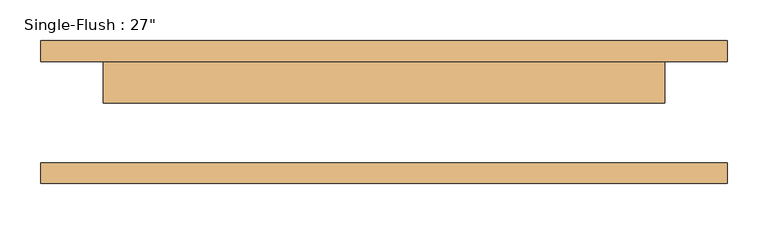
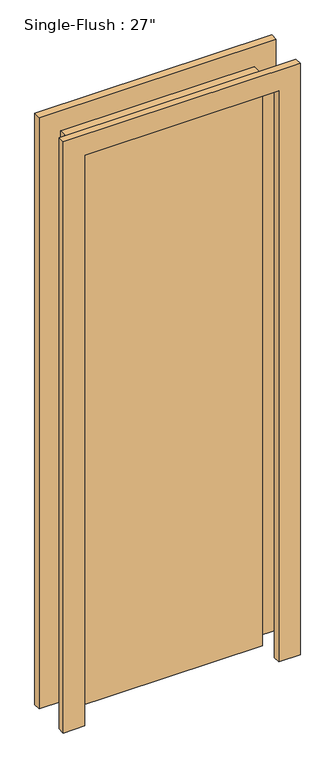
"""IFC4 building model written with IfcOpenShell, lengths in millimetres: door geometry."""

import ifcopenshell
import ifcopenshell.guid

model = None  # the IFC model being written
_history = None  # IfcOwnerHistory: only IFC2X3 demands one
_inside = {}  # id of a spatial element -> (the spatial element, [elements in it])
_under = {}  # id of a project, library or spatial element -> (it, [spatial elements below it])
_declared = {}  # id of a project -> (the project, [libraries it declares])
_typed = {}  # id of a type object -> (the type object, [elements of that type])
_made_of = {}  # id of a material, layer set ... -> (it, [elements and type objects made of it])


def new_model(schema):
    """Start an empty IFC model of exactly this schema.

    Asked for "IFC4X3", IfcOpenShell would pick the latest addendum, in which some entities
    have other attributes; the version numbers below select the first issue.
    IFC2X3 requires an IfcOwnerHistory on every rooted entity: one is made here for all.
    """
    global model, _history
    if schema == "IFC4X3":
        model = ifcopenshell.file(schema_version=(4, 3, 0, 0))
    else:
        model = ifcopenshell.file(schema=schema)
    _inside.clear()
    _under.clear()
    _declared.clear()
    _typed.clear()
    _made_of.clear()
    _history = None
    if model.schema == "IFC2X3":
        org = make("IfcOrganization", Name="unknown")
        user = make(
            "IfcPersonAndOrganization",
            ThePerson=make("IfcPerson", FamilyName="unknown"),
            TheOrganization=org,
        )
        app = make(
            "IfcApplication",
            ApplicationDeveloper=org,
            Version="unknown",
            ApplicationFullName="unknown",
            ApplicationIdentifier="unknown",
        )
        _history = make(
            "IfcOwnerHistory",
            OwningUser=user,
            OwningApplication=app,
            ChangeAction="ADDED",
            CreationDate=0,
        )
    return model


def make(cls, **values):
    """One entity of the class cls with the attributes given. An attribute that is None is left unset."""
    return model.create_entity(
        cls, **{name: value for name, value in values.items() if value is not None}
    )


def rooted(cls, **values):
    """An entity with a GlobalId (a new one), such as an element, a storey or a relation."""
    return make(cls, GlobalId=ifcopenshell.guid.new(), OwnerHistory=_history, **values)


def si_unit(unit_type, name, prefix=None):
    """IfcSIUnit, for example si_unit("LENGTHUNIT", "METRE", prefix="MILLI")."""
    return make("IfcSIUnit", UnitType=unit_type, Prefix=prefix, Name=name)


def assignment(units):
    """IfcUnitAssignment: the units of a project."""
    return None if units is None else make("IfcUnitAssignment", Units=units)


def point(xyz):
    """IfcCartesianPoint."""
    return None if xyz is None else make("IfcCartesianPoint", Coordinates=xyz)


def direction(xyz):
    """IfcDirection."""
    return None if xyz is None else make("IfcDirection", DirectionRatios=xyz)


def frame(location, z_axis=None, x_axis=None):
    """IfcAxis2Placement3D, a coordinate frame: its origin and axes. An axis left out is left unset."""
    return make(
        "IfcAxis2Placement3D",
        Location=point(location),
        Axis=direction(z_axis),
        RefDirection=direction(x_axis),
    )


def origin():
    """The frame at (0, 0, 0) with its axes left unset."""
    return frame((0.0, 0.0, 0.0))


def origin_with_axes():
    """The frame at (0, 0, 0) with the z axis (0, 0, 1) and the x axis (1, 0, 0) written out."""
    return frame((0.0, 0.0, 0.0), z_axis=(0.0, 0.0, 1.0), x_axis=(1.0, 0.0, 0.0))


def place(relative_to, where):
    """IfcLocalPlacement: puts the frame where relative to a parent placement (None: the world)."""
    return make(
        "IfcLocalPlacement", PlacementRelTo=relative_to, RelativePlacement=where
    )


def context(
    kind, dimensions, precision=None, world=None, true_north=None, identifier=None
):
    """IfcGeometricRepresentationContext, for example the 3D "Model" context."""
    return make(
        "IfcGeometricRepresentationContext",
        ContextIdentifier=identifier,
        ContextType=kind,
        CoordinateSpaceDimension=dimensions,
        Precision=precision,
        WorldCoordinateSystem=world,
        TrueNorth=true_north,
    )


def project(units=None, contexts=None):
    """IfcProject with its units and contexts."""
    return rooted(
        "IfcProject",
        Name="project",
        RepresentationContexts=contexts,
        UnitsInContext=assignment(units),
    )


def spatial(cls, under=None, at=None, **own):
    """A site, building, storey or space (cls), placed at a placement, below another one or the project."""
    s = rooted(cls, ObjectPlacement=at, **own)
    if under is not None:
        _under.setdefault(under.id(), (under, []))[1].append(s)
    return s


def polyline(points):
    """IfcPolyline through the points."""
    return make("IfcPolyline", Points=[point(p) for p in points])


def outline(outer, holes=None, kind="AREA"):
    """IfcArbitraryClosedProfileDef: a profile drawn as a closed curve; with holes, ...WithVoids."""
    if holes is None:
        return make("IfcArbitraryClosedProfileDef", ProfileType=kind, OuterCurve=outer)
    return make(
        "IfcArbitraryProfileDefWithVoids",
        ProfileType=kind,
        OuterCurve=outer,
        InnerCurves=holes,
    )


def extrude(swept, where, along, depth):
    """IfcExtrudedAreaSolid: the profile swept, set in the frame where, extruded along a direction by depth."""
    return make(
        "IfcExtrudedAreaSolid",
        SweptArea=swept,
        Position=where,
        ExtrudedDirection=direction(along),
        Depth=depth,
    )


def shape(context_of_items, identifier, shape_type, items):
    """IfcShapeRepresentation: the items that make up one representation, for example the "Body"."""
    return make(
        "IfcShapeRepresentation",
        ContextOfItems=context_of_items,
        RepresentationIdentifier=identifier,
        RepresentationType=shape_type,
        Items=items,
    )


def source(mapping_origin, context_of_items, identifier, shape_type, items):
    """IfcRepresentationMap: a shape defined once, which mapped items show again and again."""
    return make(
        "IfcRepresentationMap",
        MappingOrigin=mapping_origin,
        MappedRepresentation=shape(context_of_items, identifier, shape_type, items),
    )


def transform(
    local_origin,
    x_axis=None,
    y_axis=None,
    z_axis=None,
    scale=None,
    scale2=None,
    scale3=None,
    uniform=True,
):
    """IfcCartesianTransformationOperator3D, or its non-uniform kind. x_axis, y_axis, z_axis: its Axis1, 2, 3."""
    if uniform:
        return make(
            "IfcCartesianTransformationOperator3D",
            Axis1=direction(x_axis),
            Axis2=direction(y_axis),
            LocalOrigin=point(local_origin),
            Scale=scale,
            Axis3=direction(z_axis),
        )
    return make(
        "IfcCartesianTransformationOperator3DnonUniform",
        Axis1=direction(x_axis),
        Axis2=direction(y_axis),
        LocalOrigin=point(local_origin),
        Scale=scale,
        Axis3=direction(z_axis),
        Scale2=scale2,
        Scale3=scale3,
    )


def mapped(mapping_source, mapping_target):
    """IfcMappedItem: shows the shape of a source again, moved by a transform."""
    return make(
        "IfcMappedItem", MappingSource=mapping_source, MappingTarget=mapping_target
    )


def made_of(thing, what):
    """Note that an element or type object is made of a material, layer set ...; save() writes the relation."""
    if what is not None:
        _made_of.setdefault(what.id(), (what, []))[1].append(thing)
    return thing


def element(
    cls,
    number,
    at=None,
    inside=None,
    cuts=None,
    type_object=None,
    material=None,
    context=None,
    identifier="Body",
    shape_type=None,
    held_by="IfcProductDefinitionShape",
    body=None,
    shapes=None,
    **own,
):
    """One element of the class cls, such as IfcWall. Its Tag is "e" and its number.

    at: its placement. inside: the storey or other place that contains it. cuts: it is an
    opening in that element (IfcRelVoidsElement). A single representation is given by context,
    identifier, shape_type and body (its items); several are given by shapes. held_by: the class
    of the entity that holds the representations. save() writes the other relations.
    """
    e = rooted(cls, Tag="e%d" % number, ObjectPlacement=at, **own)
    if body is not None:
        shapes = [shape(context, identifier, shape_type, body)]
    if shapes is not None:
        e.Representation = make(held_by, Representations=shapes)
    if inside is not None:
        _inside.setdefault(inside.id(), (inside, []))[1].append(e)
    if cuts is not None:
        rooted(
            "IfcRelVoidsElement", RelatingBuildingElement=cuts, RelatedOpeningElement=e
        )
    if type_object is not None:
        _typed.setdefault(type_object.id(), (type_object, []))[1].append(e)
    return made_of(e, material)


def aggregate(whole, parts):
    """IfcRelAggregates: a whole, such as a stair, and the parts it consists of."""
    return rooted("IfcRelAggregates", RelatingObject=whole, RelatedObjects=parts)


def save(model, path):
    """Write the relations noted so far, then the file.

    IfcRelAggregates (storeys below a building ...), IfcRelContainedInSpatialStructure (elements
    in a storey), IfcRelDefinesByType, IfcRelAssociatesMaterial and IfcRelDeclares: one each for
    every whole, place, type object, material and project.
    """
    for whole, parts in _under.values():
        aggregate(whole, parts)
    for where, things in _inside.values():
        rooted(
            "IfcRelContainedInSpatialStructure",
            RelatedElements=things,
            RelatingStructure=where,
        )
    for kind, things in _typed.values():
        rooted("IfcRelDefinesByType", RelatedObjects=things, RelatingType=kind)
    for what, things in _made_of.values():
        rooted("IfcRelAssociatesMaterial", RelatedObjects=things, RelatingMaterial=what)
    for by, libraries in _declared.values():
        rooted("IfcRelDeclares", RelatingContext=by, RelatedDefinitions=libraries)
    model.write(path)


def door_3be2e7dd(model_context):
    return source(origin(), model_context, "Body", "SweptSolid", [
        extrude(outline(polyline([(2209.8, -419.1), (0.0, -419.1), (0.0, -342.9), (2133.6, -342.9), (2133.6, 342.9), (0.0, 342.9), (0.0, 419.1), (2209.8, 419.1), (2209.8, -419.1)])), frame((0.0, 61.9125, 0.0), z_axis=(0.0, 1.0, 0.0), x_axis=(0.0, 0.0, 1.0)), (0.0, 0.0, 1.0), 25.4),
        extrude(outline(polyline([(2209.8, 419.1), (2209.8, -419.1), (0.0, -419.1), (0.0, -342.9), (2133.6, -342.9), (2133.6, 342.9), (0.0, 342.9), (0.0, 419.1), (2209.8, 419.1)])), frame((0.0, -87.3125, 0.0), z_axis=(0.0, 1.0, 0.0), x_axis=(0.0, 0.0, 1.0)), (0.0, 0.0, 1.0), 25.4),
        extrude(outline(polyline([(342.9, 11.1125), (-342.9, 11.1125), (-342.9, 61.9125), (342.9, 61.9125), (342.9, 11.1125)])), origin_with_axes(), (0.0, 0.0, 1.0), 2133.6),
    ])


if __name__ == "__main__":
    model = new_model("IFC4")
    model_context = context("Model", 3, world=origin())
    ifc_project = project(units=[si_unit("LENGTHUNIT", "METRE", prefix="MILLI")], contexts=[model_context])
    site = spatial("IfcSite", under=ifc_project)
    building = spatial("IfcBuilding", under=site)
    placement = place(None, origin())
    door_shape = door_3be2e7dd(model_context)
    element("IfcDoor", 1, ObjectType="Single-Flush : 27\"", at=placement, inside=building, context=model_context, shape_type="MappedRepresentation", body=[
        mapped(door_shape, transform((0.0, 0.0, 0.0), x_axis=(1.0, 0.0, 0.0), y_axis=(0.0, 1.0, 0.0), z_axis=(0.0, 0.0, 1.0))),
    ])
    save(model, "model.ifc")

# Revit data of these elements
# Type "Single-Flush : 27\""
#   Type Mark = "55"
#   Construction Type Id = "MDOOR"
#   Assembly Code = "C1020"
#   Analytic Construction = "Metal"
#   Thickness = 0' - 2"
#   Heat Transfer Coefficient (U) = 3.7021 W/(m²·K)
#   Height = 7' - 0"
#   Trim Projection Ext = 0' - 1"
#   Trim Projection Int = 0' - 1"
#   Trim Width = 0' - 3"
#   Width = 2' - 3"
#   Door Material = Door - Panel
#   Frame Material = Door - Frame
#   Visual Light Transmittance = 0
#   Solar Heat Gain Coefficient = 0
#   Function = (empty or 0)
#   Wall Closure = (empty or 0)
# Element 1 (IfcDoor, "Single-Flush : 27\"")
#   Materials on its faces: "Door - Frame", "Door - Panel"
# Materials
#   "Door - Panel": class "Wood", colour RGB 210 159 95, transparency 0
#   "Door - Frame": class "Miscellaneous", colour RGB 118 70 51, transparency 0
